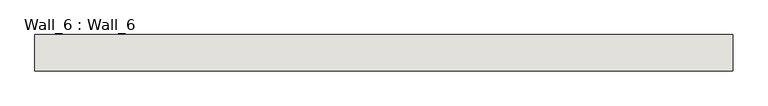
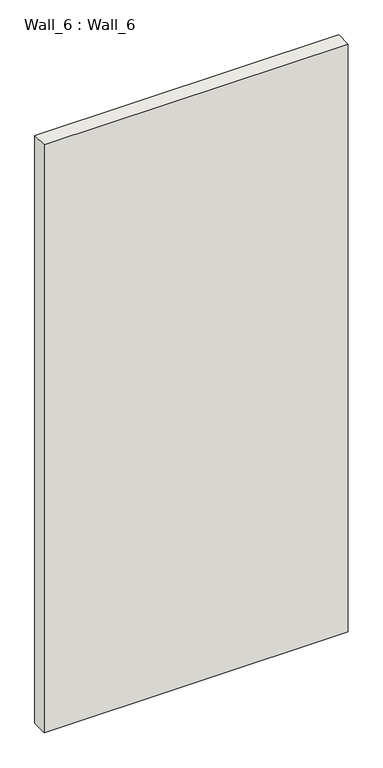
"""IFC4 building model written with IfcOpenShell, lengths in millimetres: wall geometry, Wall_6 : Wall_6."""

from ifc_helpers import new_model, si_unit, origin, origin_with_axes, place, context, project, spatial, polyline, outline, extrude, source, transform, mapped, element, save


def wall_6_wall_6_c3d1f71e(model_context):
    return source(origin(), model_context, "Body", "SweptSolid", [
        extrude(outline(polyline([(2400.0, 16870.0), (100.0, 16870.0), (100.0, 16990.0), (2400.0, 16990.0), (2400.0, 16870.0)])), origin_with_axes(), (0.0, 0.0, 1.0), 4700.0),
    ])


if __name__ == "__main__":
    model = new_model("IFC4")
    model_context = context("Model", 3, world=origin())
    ifc_project = project(units=[si_unit("LENGTHUNIT", "METRE", prefix="MILLI")], contexts=[model_context])
    site = spatial("IfcSite", under=ifc_project)
    building = spatial("IfcBuilding", under=site)
    placement = place(None, origin())
    wall_6_wall_6_shape = wall_6_wall_6_c3d1f71e(model_context)
    element("IfcWall", 1, ObjectType="Wall_6 : Wall_6", at=placement, inside=building, context=model_context, shape_type="MappedRepresentation", body=[
        mapped(wall_6_wall_6_shape, transform((0.0, 0.0, 0.0), x_axis=(1.0, 0.0, 0.0), y_axis=(0.0, 1.0, 0.0), z_axis=(0.0, 0.0, 1.0))),
    ])
    save(model, "model.ifc")

# Revit data of these elements
# Type "Wall_6 : Wall_6"
#   NameOverride = "Wall_6"
# Element 1 (IfcWall, "Wall_6 : Wall_6")
#   Materials on its faces: "IfcSurfaceStyle #33"
# Materials
#   "IfcSurfaceStyle #33": class "Unassigned", colour RGB 214 214 214, transparency 0
